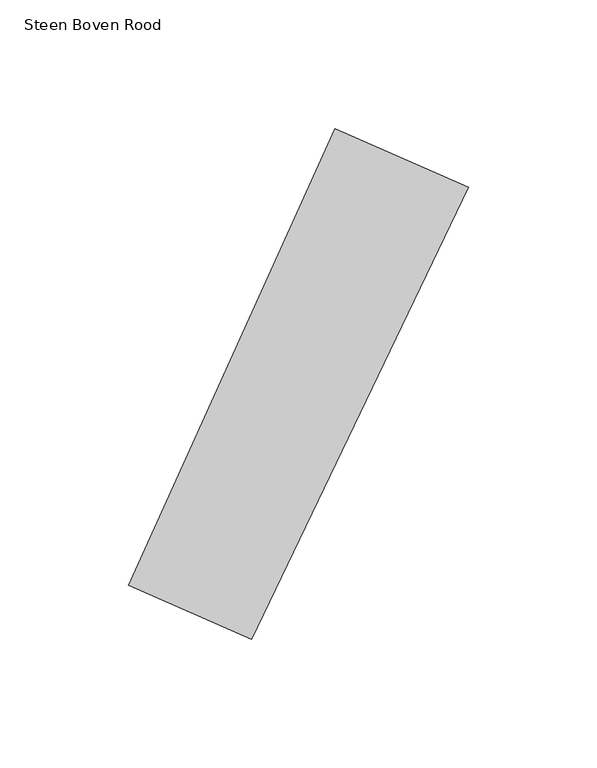
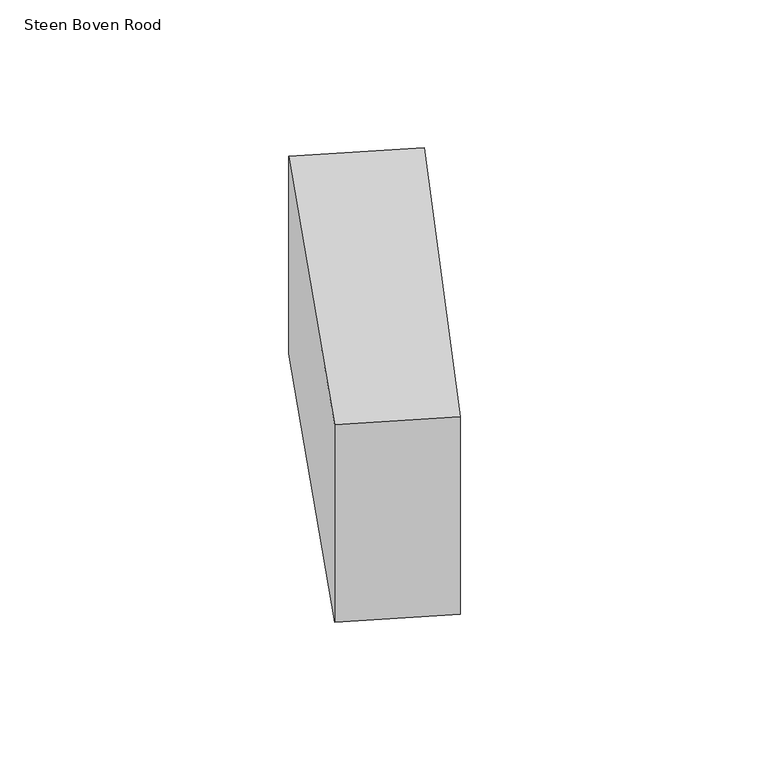
"""IFC4 building model written with IfcOpenShell, lengths in millimetres: proxy geometry, 00_GMA_steen_versie_4 : Steen Boven Rood."""

from ifc_helpers import new_model, si_unit, origin, origin_with_axes, place, context, project, spatial, polyline, outline, extrude, source, transform, mapped, element, save


def steen_boven_rood_c7edbaf4(model_context):
    return source(origin(), model_context, "Body", "SweptSolid", [
        extrude(outline(polyline([(144.2767174, 160.8094297), (59.8392253, -15.0841927), (11.9329983, 5.9814636), (92.4027419, 183.6173619), (144.2767174, 160.8094297)])), origin_with_axes(), (0.0, 0.0, 1.0), 100.0),
    ])


if __name__ == "__main__":
    model = new_model("IFC4")
    model_context = context("Model", 3, world=origin())
    ifc_project = project(units=[si_unit("LENGTHUNIT", "METRE", prefix="MILLI")], contexts=[model_context])
    site = spatial("IfcSite", under=ifc_project)
    building = spatial("IfcBuilding", under=site)
    placement = place(None, origin())
    steen_boven_rood_shape = steen_boven_rood_c7edbaf4(model_context)
    element("IfcBuildingElementProxy", 1, Name="00_GMA_steen_versie_4 : Steen Boven Rood", ObjectType="00_GMA_steen_versie_4 : Steen Boven Rood", at=placement, inside=building, context=model_context, shape_type="MappedRepresentation", body=[
        mapped(steen_boven_rood_shape, transform((0.0, 0.0, 0.0), x_axis=(1.0, 0.0, 0.0), y_axis=(0.0, 1.0, 0.0), z_axis=(0.0, 0.0, 1.0))),
    ])
    save(model, "model.ifc")

# Revit data of these elements
# Type "00_GMA_steen_versie_4 : Steen Boven Rood"
#   StootVoegHalfBoven [instance default] = 5 mm
#   StootVoegHalf [instance default] = 5 mm
#   StootVoegBreedteOnder = 10 mm
#   StootVoegBreedteBoven = 10 mm
#   Steendikte = 100 mm
#   LintVoegOnderHalf = 5 mm
#   LintVoegOnder = 10 mm
#   LintVoegBovenHalf = 0 mm
#   LintVoegBoven = 0 mm
#   materiaal = 21_steen_rood
#   MateriaalVoeg = none
#   Default Elevation = 0
# Element 1 (IfcBuildingElementProxy, "00_GMA_steen_versie_4 : Steen Boven Rood")
#   Materials on its faces: "21_steen_rood"
# Materials
#   "21_steen_rood": class "Unassigned", colour RGB 213 111 43, transparency 0, Cost = 0
